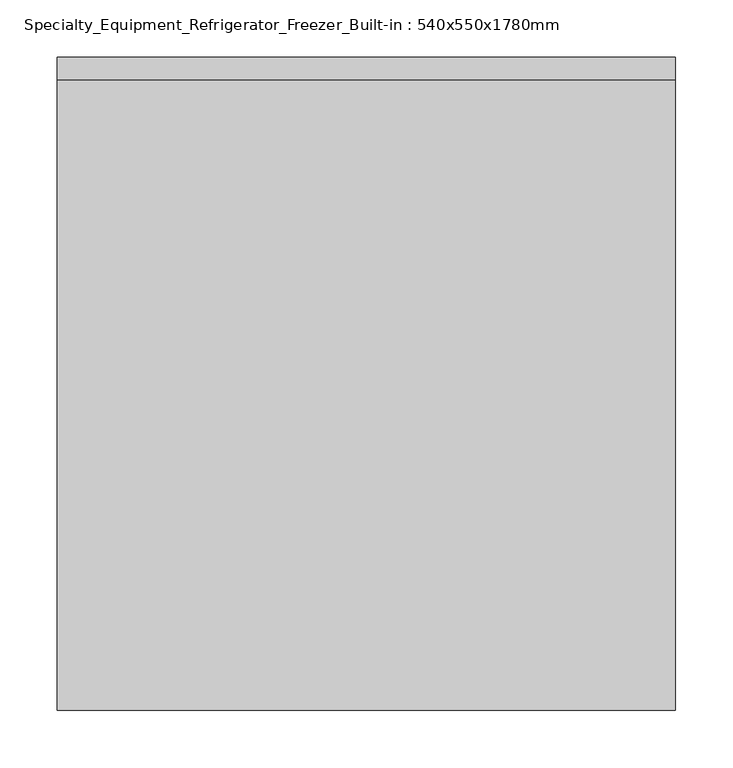
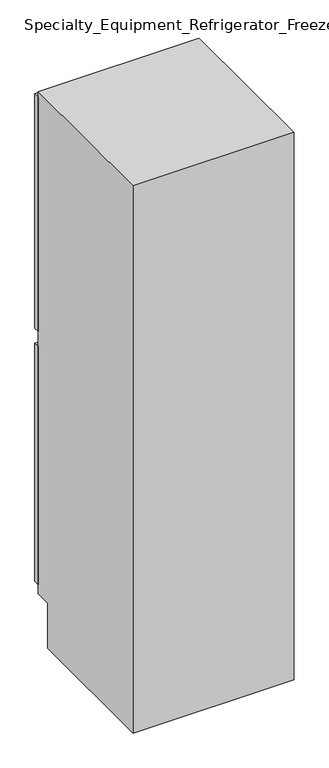
"""IFC4 building model written with IfcOpenShell, lengths in millimetres: proxy geometry, Specialty_Equipment_Refrigerator_Freezer_Built-in : 540x550x1780mm."""

from ifc_helpers import new_model, si_unit, frame, origin, place, context, project, spatial, polyline, outline, extrude, source, transform, mapped, element, save


def specialty_equipment_refrigerator_freezer_built_in_e59dad0f(model_context):
    return source(origin(), model_context, "Body", "SweptSolid", [
        extrude(outline(polyline([(-371.2552993, 786.25), (168.7447007, 786.25), (168.7447007, 766.25), (-371.2552993, 766.25), (-371.2552993, 786.25)])), frame((0.0, 0.0, 1090.0), z_axis=(0.0, 0.0, 1.0), x_axis=(1.0, 0.0, 0.0)), (0.0, 0.0, 1.0), 830.0),
        extrude(outline(polyline([(-371.2552993, 786.25), (168.7447007, 786.25), (168.7447007, 766.25), (-371.2552993, 766.25), (-371.2552993, 786.25)])), frame((0.0, 0.0, 192.0), z_axis=(0.0, 0.0, 1.0), x_axis=(1.0, 0.0, 0.0)), (0.0, 0.0, 1.0), 845.0),
        extrude(outline(polyline([(711.0710563, 0.0), (216.25, 0.0), (216.25, 1940.0), (766.25, 1940.0), (766.25, 160.0), (711.0710563, 160.0), (711.0710563, 0.0)])), frame((-371.2552993, 0.0, 0.0), z_axis=(1.0, 0.0, 0.0), x_axis=(0.0, 1.0, 0.0)), (0.0, 0.0, 1.0), 540.0),
    ])


if __name__ == "__main__":
    model = new_model("IFC4")
    model_context = context("Model", 3, world=origin())
    ifc_project = project(units=[si_unit("LENGTHUNIT", "METRE", prefix="MILLI")], contexts=[model_context])
    site = spatial("IfcSite", under=ifc_project)
    building = spatial("IfcBuilding", under=site)
    placement = place(None, origin())
    specialty_equipment_refrigerator_freezer_built_in_shape = specialty_equipment_refrigerator_freezer_built_in_e59dad0f(model_context)
    element("IfcBuildingElementProxy", 1, Name="Specialty_Equipment_Refrigerator_Freezer_Built-in : 540x550x1780mm", ObjectType="Specialty_Equipment_Refrigerator_Freezer_Built-in : 540x550x1780mm", at=placement, inside=building, context=model_context, shape_type="MappedRepresentation", body=[
        mapped(specialty_equipment_refrigerator_freezer_built_in_shape, transform((0.0, 0.0, 0.0), x_axis=(1.0, 0.0, 0.0), y_axis=(0.0, 1.0, 0.0), z_axis=(0.0, 0.0, 1.0))),
    ])
    save(model, "model.ifc")

# Revit data of these elements
# Type "Specialty_Equipment_Refrigerator_Freezer_Built-in : 540x550x1780mm"
#   Label = "REF."
#   Keynote = "N"
#   Depth = 550 mm
#   Height = 1780 mm
#   Plinth Height = 160 mm
#   Width = 540 mm
#   Material = Metal - Paint Finish - Ivory, Glossy
# Element 1 (IfcBuildingElementProxy, "Specialty_Equipment_Refrigerator_Freezer_Built-in : 540x550x1780mm")
#   Materials on its faces: "Metal - Paint Finish - Ivory, Glossy"
# Materials
#   "Metal - Paint Finish - Ivory, Glossy": class "Paint", colour RGB 247 247 239, transparency 0
